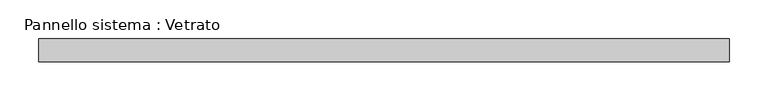
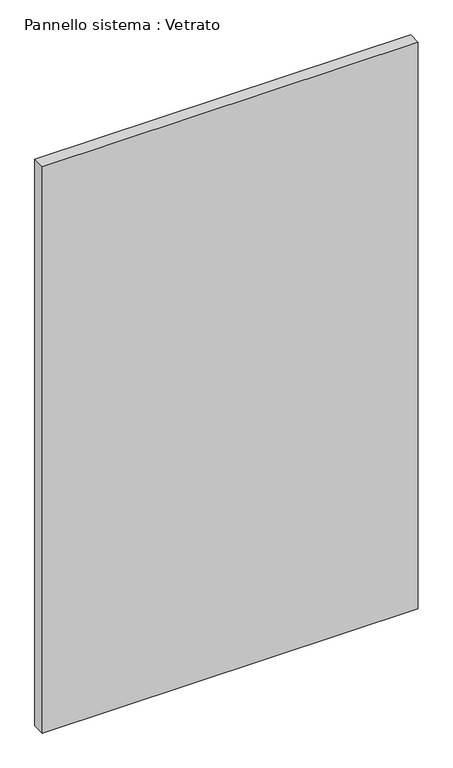
"""IFC4 building model written with IfcOpenShell, lengths in millimetres: plate geometry, Pannello sistema : Vetrato."""

from ifc_helpers import new_model, si_unit, origin, origin_with_axes, place, context, project, spatial, polyline, outline, extrude, source, transform, mapped, element, save


def pannello_sistema_vetrato_0283be3b(model_context):
    return source(origin(), model_context, "Body", "SweptSolid", [
        extrude(outline(polyline([(447.5, -15.0), (-447.5, -15.0), (-447.5, 15.0), (447.5, 15.0), (447.5, -15.0)])), origin_with_axes(), (0.0, 0.0, 1.0), 1425.0),
    ])


if __name__ == "__main__":
    model = new_model("IFC4")
    model_context = context("Model", 3, world=origin())
    ifc_project = project(units=[si_unit("LENGTHUNIT", "METRE", prefix="MILLI")], contexts=[model_context])
    site = spatial("IfcSite", under=ifc_project)
    building = spatial("IfcBuilding", under=site)
    placement = place(None, origin())
    pannello_sistema_vetrato_shape = pannello_sistema_vetrato_0283be3b(model_context)
    element("IfcPlate", 1, ObjectType="Pannello sistema : Vetrato", at=placement, inside=building, context=model_context, shape_type="MappedRepresentation", body=[
        mapped(pannello_sistema_vetrato_shape, transform((0.0, 0.0, 0.0), x_axis=(1.0, 0.0, 0.0), y_axis=(0.0, 1.0, 0.0), z_axis=(0.0, 0.0, 1.0))),
    ])
    save(model, "model.ifc")

# Revit data of these elements
# Type "Pannello sistema : Vetrato"
#   Construction Type Id = "GSP4R"
#   Analytic Construction = "Vetrata singola Pilkington 1/8 in"
#   Visual Light Transmittance = 0.9
#   Solar Heat Gain Coefficient = 0.86
#   Heat Transfer Coefficient (U) = 6.7069 W/(m²·K)
# Element 1 (IfcPlate, "Pannello sistema : Vetrato")
#   Materials on its faces: "Default - Vetro"
# Materials
#   "Default - Vetro": class "Vetro", colour RGB 208 208 208, transparency 0.7, Cost = 0
